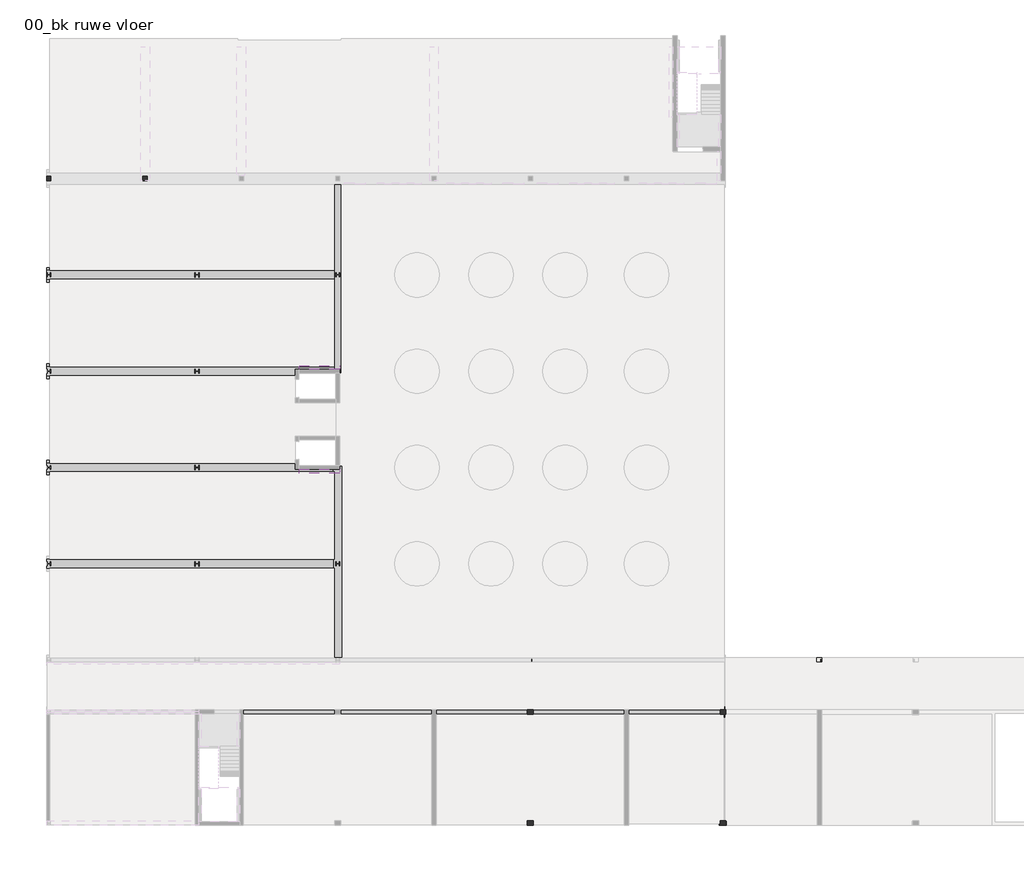
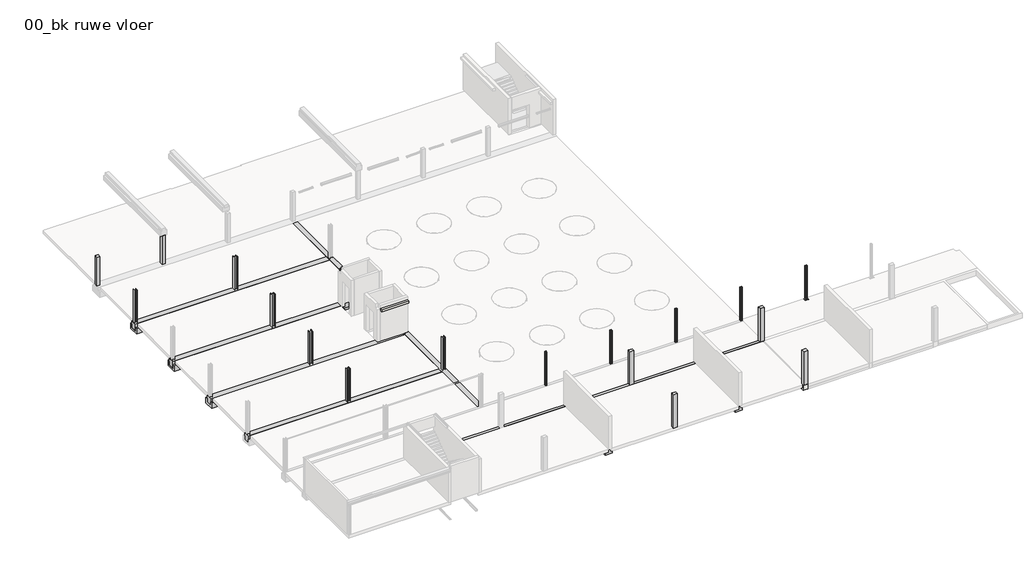
# One storey, part 5 of 6: 17 columns, 12 beams, 2 footings, 2 walls.
# Revit data of these elements (continued)
# Type "NLRS_28_SF_LIB_balk dubbele sponning beton ihwg-CWV-MMBC-SRP_gen_rsf : balk beton ihwg_gen__bxh 900x900 met inkassing bxh 200x320" (continued)
#   RSF_C_breedte_inkassing_rechts = 200 mm
#   RSF_C_breedte_inkassing_links = 200 mm
#   NLRS_C_lengte [instance default] = 3000 mm
#   NLRS_C_hoogte = 900 mm
#   NLRS_C_breedte = 900 mm
#   Length [instance default] = 3000 mm
#   Structural Material = NLRS_f2_beton ihwg_gen_rsf
#   Model = ""
# Type "NLRS_28_SCO_TLB_stalen kolom HEA-BCPG-MMBS-SRP_gen_rsf : stalen kolom_gen__HEA 260"
#   Type IfcGUID = "2$hNzCXOT3YR8V$0CfyzGd"
#   IfcExportAs = "IfcColumnType"
#   IfcExportType = "COLUMN"
#   Type Comments = "HEA260"
#   Model = " "
#   Manufacturer = " "
#   Description = "stalen kolom HEA260"
#   Assembly Code = "28.11"
#   vz = 125 mm
#   vy = 130 mm
#   vpz = 125 mm
#   vpy = 130 mm
#   tw = 7.5 mm
#   tf = 12.5 mm
#   ra = 24 mm
#   d = 250 mm
#   bf = 260 mm
#   NLRS_C_lengte [instance default] = 2743.2 mm
#   Structural Material = NLRS_h2_staal_gen_rsf
#   Keynote = ""
# Type "NLRS_28_SCO_TLB_vierkante kolom beton prefab-BCPG-MMBPC-SRP_gen_rsf : kolom vierkant beton prefab_gen__bxh 300x300"
#   Type IfcGUID = "2bNskL0kfByRmbY5G6If0x"
#   IfcExportAs = "IfcColumnType"
#   IfcExportType = "COLUMN"
#   Type Comments = "300x300"
#   Model = "LOD300"
#   Description = "prefab betonkolom 300x300"
#   Assembly Code = "28.11"
#   NLRS_C_lengte [instance default] = 2700 mm
#   NLRS_C_hoogte = 300 mm
#   NLRS_C_breedte = 300 mm
#   Structural Material = NLRS_f2_beton prefab_gen_rsf
# Type "NLRS_28_SCO_TLB_stalen kolom HEB-BCPG-MMBS-SRP_gen_rsf : stalen kolom_gen__HEB 300"
#   Type IfcGUID = "3C_b5Xdrv818Ti1jf59K4n"
#   IfcExportAs = "IfcColumnType"
#   IfcExportType = "COLUMN"
#   Type Comments = "HEB300"
#   Model = " "
#   Manufacturer = " "
#   Description = "stalen kolom HEB300"
#   Assembly Code = "28.11"
#   vz = 150 mm
#   vy = 150 mm
#   vpz = 150 mm
#   vpy = 150 mm
#   tw = 11 mm
#   tf = 19 mm
#   ra = 27 mm
#   d = 300 mm
#   bf = 300 mm
#   NLRS_C_lengte [instance default] = 2743.2 mm
#   Structural Material = NLRS_h2_staal_gen_rsf
#   Keynote = ""
# Type "NLRS_28_SCO_TLB_vierkante kolom beton ihwg-BCPG-MMBC-SRP_gen_rsf : vierkante kolom beton ihwg_gen__bxh 400x300"
#   Type IfcGUID = "2lw04Qbvr9TgC3fLWwYn2N"
#   IfcExportAs = "IfcColumnType"
#   IfcExportType = "COLUMN"
#   Type Comments = "400x300"
#   Model = "LOD300"
#   Description = "betonkolom ihwg 400x300"
#   Assembly Code = "28.11"
#   NLRS_C_lengte [instance default] = 2700 mm
#   NLRS_C_hoogte = 300 mm
#   NLRS_C_breedte = 400 mm
#   Structural Material = NLRS_f2_beton ihwg_gen_rsf
# Type "NLRS_28_SCO_TLB_stalen kolom buisprofiel koudgevormd vierkant-BCPG-MMBS-SRP_gen_rsf : stalen kolom buisprofiel koudgevormd vierkant RHSC_gen__160x160x8"
#   Type IfcGUID = "2$hNzCXOT3YR8V$0Cfyzxk"
#   IfcExportAs = "IfcColumnType"
#   IfcExportType = "COLUMN"
#   Type Comments = "K160x160x8"
#   Model = " "
#   Manufacturer = " "
#   Description = "stalen kolom K160x160x8"
#   Assembly Code = "28.11"
#   vz = 80 mm
#   vy = 80 mm
#   vpz = 80 mm
#   vpy = 80 mm
#   tw = 8 mm
#   tf = 8 mm
#   ri = 20 mm
#   ra = 12 mm
#   d = 160 mm
#   bf = 160 mm
#   NLRS_C_lengte [instance default] = 2743.2 mm
#   Structural Material = NLRS_h2_staal_gen_rsf
#   Keynote = ""
# Type "NLRS_16_SFO_WPB_stiep rechthoek beton ihwg-AV-MMBC_gen_rsf : stiep beton ihwg_gen__bxl 300x400"
#   IfcExportAs = "IfcFootingType"
#   Type Comments = "stiep 300x400"
#   Description = "stiep 300x400"
#   Assembly Code = "16.13"
#   Width = 300 mm
#   NLRS_C_lengte = 400 mm
#   NLRS_C_hoogte [instance default] = 600 mm
#   NLRS_C_breedte = 300 mm
#   Length = 400 mm
#   Structural Material = NLRS_f2_beton ihwg_gen_rsf
#   Model = ""
#   Default Elevation = 0
# Type "NLRS_16_SFO_WPB_stiep rechthoek beton ihwg-AV-MMBC_gen_rsf : stiep beton ihwg_gen__bxl 300x500"
#   IfcExportAs = "IfcFootingType"
#   Type Comments = "stiep 300x500"
#   Description = "stiep 300x500"
#   Assembly Code = "16.13"
#   Width = 300 mm
#   NLRS_C_lengte = 500 mm
#   NLRS_C_hoogte [instance default] = 600 mm
#   NLRS_C_breedte = 300 mm
#   Length = 500 mm
#   Structural Material = NLRS_f2_beton ihwg_gen_rsf
#   Model = ""
#   Default Elevation = 0
# Type "NLRS_22_SF_LIB_oplegnok beton prefab framing-CWV-MMBPC-SRP_gen_rsf : oplegnok beton prefab_gen__bxh 250x250/220"
#   Type IfcGUID = "3EzArCxHzFqA2seU7O0xFZ"
#   IfcExportAs = "IfcWallType"
#   Type Comments = "oplegnok"
#   Model = "LOD300"
#   Description = "oplegnok beton prefab 250x250/220"
#   Assembly Code = "22.11"
#   NLRS_C_hoogte_01 = 220 mm
#   NLRS_C_hoogte = 250 mm
#   NLRS_C_breedte = 250 mm
#   Lossing = 30 mm
#   Length [instance default] = 3000 mm
#   Structural Material = NLRS_f2_beton prefab_gen_rsf
# Element 1 (IfcBeam, "NLRS_28_SF_LIB_balk dubbele sponning beton prefab-CWV-MMBC-SRP_gen_rsf : balk beton prefab_gen__bxh 700x700 met inkassing bxh 200x320")
#   IfcGUID = "0AFZSao6j3uApvehgmz3fE"
#   NLRS_C_lengte = 32650 mm
#   IsExternal = yes
#   LoadBearing = yes
#   Phase Created = NLRS_nieuw
#   Materials on its faces: "NLRS_f2_beton prefab_gen_rsf", "NLRS_f2_beton ihwg_gen_rsf"
# Element 2 (IfcBeam, "NLRS_28_SF_LIB_balk dubbele sponning beton ihwg-CWV-MMBC-SRP_gen_rsf : balk beton ihwg_gen__bxh 1000x900 met inkassing bxh 200x320")
#   IfcGUID = "2fqjgN40rEBBKvfwcj0B$q"
#   NLRS_C_lengte = 19900 mm
#   IsExternal = yes
#   LoadBearing = yes
#   Phase Created = NLRS_nieuw
#   Materials on its faces: "NLRS_f2_beton ihwg_gen_rsf"
# Element 3 (IfcBeam, "NLRS_28_SF_LIB_balk dubbele sponning beton ihwg-CWV-MMBC-SRP_gen_rsf : balk beton ihwg_gen__bxh 1000x900 met inkassing bxh 200x320")
#   IfcGUID = "2fqjgN40rEBBKvfwcj0Bzp"
#   NLRS_C_lengte = 19400 mm
#   IsExternal = yes
#   LoadBearing = yes
#   Phase Created = NLRS_nieuw
#   Materials on its faces: "NLRS_f2_beton ihwg_gen_rsf"
# Element 4 (IfcBeam, "NLRS_28_SF_LIB_balk dubbele sponning beton ihwg-CWV-MMBC-SRP_gen_rsf : balk beton ihwg_gen__bxh 1000x900 met inkassing bxh 200x320")
#   IfcGUID = "2fqjgN40rEBBKvfwcj0BzL"
#   NLRS_C_lengte = 19400 mm
#   IsExternal = yes
#   LoadBearing = yes
#   Phase Created = NLRS_nieuw
#   Materials on its faces: "NLRS_f2_beton ihwg_gen_rsf"
# Element 5 (IfcBeam, "NLRS_28_SF_LIB_balk dubbele sponning beton ihwg-CWV-MMBC-SRP_gen_rsf : balk beton ihwg_gen__bxh 1000x900 met inkassing bxh 200x320")
#   IfcGUID = "2fqjgN40rEBBKvfwcj0BY9"
#   NLRS_C_lengte = 19900 mm
#   IsExternal = yes
#   LoadBearing = yes
#   Phase Created = NLRS_nieuw
#   Materials on its faces: "NLRS_f2_beton ihwg_gen_rsf"
# Element 6 (IfcBeam, "NLRS_28_SF_LIB_balkbodem beton prefab-CWV-MMBC-SRP_gen_rsf : balkbodem beton prefab_gen__bxhxdk 1000x580x200")
#   IfcGUID = "0X0KViByb4JPBOa4XaNhJF"
#   NLRS_C_lengte = 19200 mm
#   IsExternal = yes
#   LoadBearing = yes
#   Phase Created = NLRS_nieuw
#   Materials on its faces: "NLRS_f2_beton prefab_gen_rsf"
# Element 7 (IfcBeam, "NLRS_28_SF_LIB_balkbodem beton prefab-CWV-MMBC-SRP_gen_rsf : balkbodem beton prefab_gen__bxhxdk 1000x580x200")
#   IfcGUID = "0X0KViByb4JPBOa4XaNgQF"
#   NLRS_C_lengte = 19200 mm
#   IsExternal = yes
#   LoadBearing = yes
#   Phase Created = NLRS_nieuw
#   Materials on its faces: "NLRS_f2_beton prefab_gen_rsf", "NLRS_f2_beton ihwg_gen_rsf"
# Element 8 (IfcBeam, "NLRS_28_SF_LIB_balkbodem beton prefab-CWV-MMBC-SRP_gen_rsf : balkbodem beton prefab_gen__bxhxdk 1000x580x200")
#   IfcGUID = "0X0KViByb4JPBOa4XaNgQc"
#   NLRS_C_lengte = 19200 mm
#   IsExternal = yes
#   LoadBearing = yes
#   Phase Created = NLRS_nieuw
#   Materials on its faces: "NLRS_f2_beton prefab_gen_rsf", "NLRS_f2_beton ihwg_gen_rsf"
# Element 9 (IfcBeam, "NLRS_28_SF_LIB_balk dubbele sponning beton ihwg-CWV-MMBC-SRP_gen_rsf : balk beton ihwg_gen__bxh 900x900 met inkassing bxh 200x320")
#   IfcGUID = "1E6t7WhRf97hJGfj3Bm3as"
#   NLRS_C_lengte = 12725 mm
#   IsExternal = yes
#   LoadBearing = yes
#   Phase Created = NLRS_nieuw
#   Materials on its faces: "NLRS_f2_beton ihwg_gen_rsf", "NLRS_f2_beton prefab_gen_rsf"
# Element 10 (IfcBeam, "NLRS_28_SF_LIB_balk dubbele sponning beton ihwg-CWV-MMBC-SRP_gen_rsf : balk beton ihwg_gen__bxh 1000x900 met inkassing bxh 200x320")
#   IfcGUID = "3iyfZByB98yevaQCZKiCcH"
#   NLRS_C_lengte = 12975 mm
#   IsExternal = yes
#   LoadBearing = yes
#   Phase Created = NLRS_nieuw
#   Materials on its faces: "NLRS_f2_beton ihwg_gen_rsf", "NLRS_f2_beton prefab_gen_rsf"
# Element 11 (IfcBeam, "NLRS_28_SF_LIB_balk dubbele sponning beton prefab-CWV-MMBC-SRP_gen_rsf : balk beton prefab_gen__bxh 700x700 met inkassing bxh 200x320")
#   IfcGUID = "3B2jA7IzvC4Aqddp_xdWat"
#   NLRS_C_lengte = 7500 mm
#   IsExternal = yes
#   LoadBearing = yes
#   Phase Created = NLRS_nieuw
#   Materials on its faces: "NLRS_f2_beton prefab_gen_rsf", "NLRS_f2_beton ihwg_gen_rsf"
# Element 12 (IfcBeam, "NLRS_28_SF_LIB_balk dubbele sponning beton prefab-CWV-MMBC-SRP_gen_rsf : balk beton prefab_gen__bxh 700x700 met inkassing bxh 200x320")
#   IfcGUID = "3B2jA7IzvC4Aqddp_xdWZ5"
#   NLRS_C_lengte = 7500 mm
#   IsExternal = yes
#   LoadBearing = yes
#   Phase Created = NLRS_nieuw
#   Materials on its faces: "NLRS_f2_beton prefab_gen_rsf", "NLRS_f2_beton ihwg_gen_rsf"
# Element 13 (IfcColumn, "NLRS_28_SCO_TLB_stalen kolom HEA-BCPG-MMBS-SRP_gen_rsf : stalen kolom_gen__HEA 260")
#   IfcGUID = "2$hNzCXOT3YR8V$0Cfyz1k"
#   Comments = ""
#   IsExternal = no
#   LoadBearing = yes
#   Phase Created = NLRS_nieuw
#   Materials on its faces: "NLRS_h2_staal_gen_rsf"
# Element 14 (IfcColumn, "NLRS_28_SCO_TLB_vierkante kolom beton prefab-BCPG-MMBPC-SRP_gen_rsf : kolom vierkant beton prefab_gen__bxh 300x300")
#   IfcGUID = "2$hNzCXOT3YR8V$0CfyzES"
#   IsExternal = no
#   LoadBearing = yes
#   Phase Created = NLRS_nieuw
#   Materials on its faces: "NLRS_f2_beton prefab_gen_rsf"
# Element 15 (IfcColumn, "NLRS_28_SCO_TLB_vierkante kolom beton prefab-BCPG-MMBPC-SRP_gen_rsf : kolom vierkant beton prefab_gen__bxh 300x300")
#   IfcGUID = "2ajLwCSRTE_9I1Spg4tpgS"
#   IsExternal = no
#   LoadBearing = yes
#   Phase Created = NLRS_nieuw
#   Materials on its faces: "NLRS_f2_beton prefab_gen_rsf"
# Element 16 (IfcColumn, "NLRS_28_SCO_TLB_stalen kolom HEB-BCPG-MMBS-SRP_gen_rsf : stalen kolom_gen__HEB 300")
#   IfcGUID = "2GRbcre991teoKeCLB8Lxx"
#   Comments = ""
#   IsExternal = no
#   LoadBearing = yes
#   Phase Created = NLRS_nieuw
#   Materials on its faces: "NLRS_h2_staal_gen_rsf"
# Element 17 (IfcColumn, "NLRS_28_SCO_TLB_stalen kolom HEB-BCPG-MMBS-SRP_gen_rsf : stalen kolom_gen__HEB 300")
#   IfcGUID = "2GRbcre991teoKeCLB8Lxv"
#   Comments = ""
#   IsExternal = no
#   LoadBearing = yes
#   Phase Created = NLRS_nieuw
#   Materials on its faces: "NLRS_h2_staal_gen_rsf"
# Element 18 (IfcColumn, "NLRS_28_SCO_TLB_stalen kolom HEB-BCPG-MMBS-SRP_gen_rsf : stalen kolom_gen__HEB 300")
#   IfcGUID = "2GRbcre991teoKeCLB8Lxd"
#   Comments = ""
#   IsExternal = no
#   LoadBearing = yes
#   Phase Created = NLRS_nieuw
#   Materials on its faces: "NLRS_h2_staal_gen_rsf"
# Element 19 (IfcColumn, "NLRS_28_SCO_TLB_stalen kolom HEB-BCPG-MMBS-SRP_gen_rsf : stalen kolom_gen__HEB 300")
#   IfcGUID = "2GRbcre991teoKeCLB8Lxb"
#   Comments = ""
#   IsExternal = no
#   LoadBearing = yes
#   Phase Created = NLRS_nieuw
#   Materials on its faces: "NLRS_h2_staal_gen_rsf"
# Element 20 (IfcColumn, "NLRS_28_SCO_TLB_stalen kolom HEA-BCPG-MMBS-SRP_gen_rsf : stalen kolom_gen__HEA 260")
#   IfcGUID = "2GRbcre991teoKeCLB8Lwq"
#   Comments = ""
#   IsExternal = no
#   LoadBearing = yes
#   Phase Created = NLRS_nieuw
#   Materials on its faces: "NLRS_h2_staal_gen_rsf"
# Element 21 (IfcColumn, "NLRS_28_SCO_TLB_vierkante kolom beton ihwg-BCPG-MMBC-SRP_gen_rsf : vierkante kolom beton ihwg_gen__bxh 400x300")
#   IfcGUID = "2lw04Qbvr9TgC3fLWwYn7K"
#   IsExternal = no
#   LoadBearing = yes
#   Phase Created = NLRS_nieuw
#   Materials on its faces: "NLRS_f2_beton ihwg_gen_rsf"
# Element 22 (IfcColumn, "NLRS_28_SCO_TLB_vierkante kolom beton ihwg-BCPG-MMBC-SRP_gen_rsf : vierkante kolom beton ihwg_gen__bxh 400x300")
#   IfcGUID = "2lw04Qbvr9TgC3fLWwYn61"
#   IsExternal = no
#   LoadBearing = yes
#   Phase Created = NLRS_nieuw
#   Materials on its faces: "NLRS_f2_beton ihwg_gen_rsf"
# Element 23 (IfcColumn, "NLRS_28_SCO_TLB_vierkante kolom beton ihwg-BCPG-MMBC-SRP_gen_rsf : vierkante kolom beton ihwg_gen__bxh 400x300")
#   IfcGUID = "2lw04Qbvr9TgC3fLWwYn5w"
#   IsExternal = no
#   LoadBearing = yes
#   Phase Created = NLRS_nieuw
#   Materials on its faces: "NLRS_f2_beton ihwg_gen_rsf"
# Element 24 (IfcColumn, "NLRS_28_SCO_TLB_vierkante kolom beton ihwg-BCPG-MMBC-SRP_gen_rsf : vierkante kolom beton ihwg_gen__bxh 400x300")
#   IfcGUID = "2lw04Qbvr9TgC3fLWwYn5T"
#   IsExternal = no
#   LoadBearing = yes
#   Phase Created = NLRS_nieuw
#   Materials on its faces: "NLRS_f2_beton ihwg_gen_rsf"
# Element 25 (IfcColumn, "NLRS_28_SCO_TLB_stalen kolom buisprofiel koudgevormd vierkant-BCPG-MMBS-SRP_gen_rsf : stalen kolom buisprofiel koudgevormd vierkant RHSC_gen__160x160x8")
#   IfcGUID = "2$hNzCXOT3YR8V$0Cfyzu5"
#   IsExternal = no
#   LoadBearing = yes
#   Phase Created = NLRS_nieuw
#   Materials on its faces: "NLRS_h2_staal_gen_rsf"
# Element 26 (IfcColumn, "NLRS_28_SCO_TLB_stalen kolom buisprofiel koudgevormd vierkant-BCPG-MMBS-SRP_gen_rsf : stalen kolom buisprofiel koudgevormd vierkant RHSC_gen__160x160x8")
#   IfcGUID = "2$hNzCXOT3YR8V$0Cfyzb1"
#   IsExternal = no
#   LoadBearing = yes
#   Phase Created = NLRS_nieuw
#   Materials on its faces: "NLRS_h2_staal_gen_rsf"
# Element 27 (IfcColumn, "NLRS_28_SCO_TLB_stalen kolom buisprofiel koudgevormd vierkant-BCPG-MMBS-SRP_gen_rsf : stalen kolom buisprofiel koudgevormd vierkant RHSC_gen__160x160x8")
#   IfcGUID = "2$hNzCXOT3YR8V$0CfyzZS"
#   IsExternal = no
#   LoadBearing = yes
#   Phase Created = NLRS_nieuw
#   Materials on its faces: "NLRS_h2_staal_gen_rsf"
# Element 28 (IfcColumn, "NLRS_28_SCO_TLB_stalen kolom buisprofiel koudgevormd vierkant-BCPG-MMBS-SRP_gen_rsf : stalen kolom buisprofiel koudgevormd vierkant RHSC_gen__160x160x8")
#   IfcGUID = "2$hNzCXOT3YR8V$0CfyzXQ"
#   IsExternal = no
#   LoadBearing = yes
#   Phase Created = NLRS_nieuw
#   Materials on its faces: "NLRS_h2_staal_gen_rsf"
# Element 29 (IfcColumn, "NLRS_28_SCO_TLB_stalen kolom buisprofiel koudgevormd vierkant-BCPG-MMBS-SRP_gen_rsf : stalen kolom buisprofiel koudgevormd vierkant RHSC_gen__160x160x8")
#   IfcGUID = "2$hNzCXOT3YR8V$0CfyzlM"
#   IsExternal = no
#   LoadBearing = yes
#   Phase Created = NLRS_nieuw
#   Materials on its faces: "NLRS_h2_staal_gen_rsf"
# Element 30 (IfcFooting, "NLRS_16_SFO_WPB_stiep rechthoek beton ihwg-AV-MMBC_gen_rsf : stiep beton ihwg_gen__bxl 300x400")
#   IfcGUID = "3aMdMHoe12P9KDGPyaIelA"
#   NLRS_C_hoogte = 520 mm
#   IsExternal = yes
#   LoadBearing = yes
#   Phase Created = NLRS_nieuw
#   Materials on its faces: "NLRS_f2_beton ihwg_gen_rsf"
# Element 31 (IfcFooting, "NLRS_16_SFO_WPB_stiep rechthoek beton ihwg-AV-MMBC_gen_rsf : stiep beton ihwg_gen__bxl 300x500")
#   IfcGUID = ""
#   NLRS_C_hoogte = 520 mm
#   IsExternal = yes
#   LoadBearing = yes
#   Phase Created = NLRS_nieuw
#   Materials on its faces: "NLRS_f2_beton ihwg_gen_rsf"
# Element 32 (IfcWall, "NLRS_22_SF_LIB_oplegnok beton prefab framing-CWV-MMBPC-SRP_gen_rsf : oplegnok beton prefab_gen__bxh 250x250/220")
#   IfcGUID = "0zo1UjqZ91lRsfCKsOObF0"
#   IsExternal = no
#   LoadBearing = yes
#   Phase Created = NLRS_nieuw
#   Materials on its faces: "NLRS_f2_beton prefab_gen_rsf"
# Element 33 (IfcWall, "NLRS_22_SF_LIB_oplegnok beton prefab framing-CWV-MMBPC-SRP_gen_rsf : oplegnok beton prefab_gen__bxh 250x250/220")
#   IfcGUID = "0zo1UjqZ91lRsfCKsOObqD"
#   IsExternal = no
#   LoadBearing = yes
#   Phase Created = NLRS_nieuw
#   Materials on its faces: "NLRS_f2_beton prefab_gen_rsf"
# Materials
#   "NLRS_f2_beton prefab_gen_rsf": class "F - Niet gebakken kunststeen", colour RGB 129 133 118, transparency 0, Keynote = "f2", Manufacturer = "Revit Standards Foundation", URL = "www.revitstandards.org", Description = "beton prefab", Cost = 0
#   "NLRS_f2_beton ihwg_gen_rsf": class "F - Niet gebakken kunststeen", colour RGB 129 133 118, transparency 0, Keynote = "f2", Manufacturer = "Revit Standards Foundation", URL = "www.revitstandards.org", Description = "beton ihwg", Cost = 0
#   "NLRS_h2_staal_gen_rsf": class "H - Metaal", colour RGB 189 187 185, transparency 0, Keynote = "h2", Manufacturer = "Revit Standards Foundation", URL = "www.revitstandards.org", Description = "staal", Cost = 0
